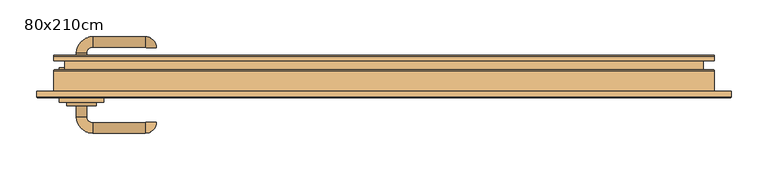
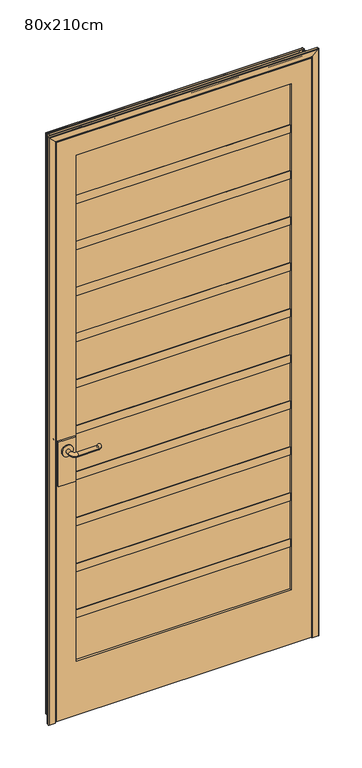
"""IFC4 building model written with IfcOpenShell, lengths in millimetres: door geometry, Porta de Abrir Metálica Quadriculada : 80x210cm."""

from ifc_helpers import new_model, si_unit, point, frame, frame_2d, origin, place, context, project, spatial, polyline, circle_curve, ellipse_curve, trimmed, segment, composite_curve, outline, extrude, source, transform, mapped, element, save
from ifc_brep_helpers import plane_surface, cylinder_surface, revolved_surface, advanced_brep


def door_80x210cm_43d22828(model_context):
    return source(origin(), model_context, "Body", "SolidModel", [
        extrude(outline(composite_curve([segment(trimmed(circle_curve(frame_2d((1050.0, -412.0)), 20.0), [point((1050.0, -432.0))], [point((1050.0, -392.0))], False, "CARTESIAN"), True, "CONTINUOUS"), segment(trimmed(circle_curve(frame_2d((1050.0, -412.0)), 20.0), [point((1050.0, -392.0))], [point((1050.0, -432.0))], False, "CARTESIAN"), True, "CONTINUOUS")], self_intersect=False)), frame((0.0, -53.6, 0.0), z_axis=(0.0, 1.0, 0.0), x_axis=(0.0, 0.0, 1.0)), (0.0, 0.0, 1.0), 4.5929895),
        advanced_brep(
        [(-405.0, -49.0070105, 1050.0), (-419.0, -49.0070105, 1050.0), (-405.0, -33.6, 1050.0), (-419.0, -33.6, 1050.0), (-397.0, -11.6, 1050.0), (-397.0, -25.6, 1050.0), (-325.0, -25.6, 1050.0), (-325.0, -11.6, 1050.0), (-324.0, -26.6, 1050.0), (-310.0, -26.6, 1050.0)],
        [
            (0, 1, circle_curve(frame((-412.0, -49.0070105, 1050.0), z_axis=(0.0, -1.0, 0.0), x_axis=(-1.0, 0.0, 0.0)), 7.0)),
            (1, 0, circle_curve(frame((-412.0, -49.0070105, 1050.0), z_axis=(0.0, -1.0, 0.0), x_axis=(-1.0, 0.0, 0.0)), 7.0)),
            (0, 2),
            (2, 3, circle_curve(frame((-412.0, -33.6, 1050.0), z_axis=(0.0, -1.0, 0.0), x_axis=(-1.0, 0.0, 0.0)), 7.0)),
            (3, 1),
            (3, 2, circle_curve(frame((-412.0, -33.6, 1050.0), z_axis=(0.0, -1.0, 0.0), x_axis=(-1.0, 0.0, 0.0)), 7.0)),
            (4, 3, circle_curve(frame((-397.0, -33.6, 1050.0), z_axis=(0.0, 0.0, 1.0), x_axis=(-1.0, 0.0, 0.0)), 22.0)),
            (2, 5, circle_curve(frame((-397.0, -33.6, 1050.0), z_axis=(0.0, 0.0, -1.0), x_axis=(-1.0, 0.0, 0.0)), 8.0)),
            (5, 4, circle_curve(frame((-397.0, -18.6, 1050.0), z_axis=(-1.0, 0.0, 0.0), x_axis=(0.0, 1.0, 0.0)), 7.0)),
            (4, 5, circle_curve(frame((-397.0, -18.6, 1050.0), z_axis=(-1.0, 0.0, 0.0), x_axis=(0.0, 1.0, 0.0)), 7.0)),
            (5, 6),
            (6, 7, circle_curve(frame((-325.0, -18.6, 1050.0), z_axis=(-1.0, 0.0, 0.0), x_axis=(0.0, 1.0, 0.0)), 7.0)),
            (7, 4),
            (7, 6, circle_curve(frame((-325.0, -18.6, 1050.0), z_axis=(-1.0, 0.0, 0.0), x_axis=(0.0, 1.0, 0.0)), 7.0)),
            (8, 9, circle_curve(frame((-317.0, -26.6, 1050.0), z_axis=(0.0, -1.0, 0.0), x_axis=(1.0, 0.0, 0.0)), 7.0)),
            (9, 8, circle_curve(frame((-317.0, -26.6, 1050.0), z_axis=(0.0, -1.0, 0.0), x_axis=(1.0, 0.0, 0.0)), 7.0)),
            (9, 7, circle_curve(frame((-325.0, -26.6, 1050.0), z_axis=(0.0, 0.0, 1.0), x_axis=(0.0, 1.0, 0.0)), 15.0)),
            (6, 8, circle_curve(frame((-325.0, -26.6, 1050.0), z_axis=(0.0, 0.0, -1.0), x_axis=(0.0, 1.0, 0.0)), 1.0)),
        ],
        [
            plane_surface(frame((-412.0, -49.0070105, 1050.0), z_axis=(0.0, -1.0, 0.0), x_axis=(0.0, 0.0, 1.0))),
            cylinder_surface(frame((-412.0, -49.0070105, 1050.0), z_axis=(0.0, -1.0, 0.0), x_axis=(-1.0, 0.0, 0.0)), 7.0),
            revolved_surface(trimmed(ellipse_curve(frame((-412.0, -33.6, 1050.0), z_axis=(0.0, -1.0, 0.0), x_axis=(-1.0, 0.0, 0.0)), 7.0, 7.0), [point((-405.0, -33.6, 1050.0))], [point((-419.0, -33.6, 1050.0))], True, "CARTESIAN"), (-397.0, -33.6, 1050.0), (0.0, 0.0, -1.0)),
            revolved_surface(trimmed(ellipse_curve(frame((-412.0, -33.6, 1050.0), z_axis=(0.0, -1.0, 0.0), x_axis=(-1.0, 0.0, 0.0)), 7.0, 7.0), [point((-419.0, -33.6, 1050.0))], [point((-405.0, -33.6, 1050.0))], True, "CARTESIAN"), (-397.0, -33.6, 1050.0), (0.0, 0.0, -1.0)),
            cylinder_surface(frame((-397.0, -18.6, 1050.0), z_axis=(-1.0, 0.0, 0.0), x_axis=(0.0, 1.0, 0.0)), 7.0),
            plane_surface(frame((-317.0, -26.6, 1050.0), z_axis=(0.0, -1.0, 0.0), x_axis=(0.0, 0.0, 1.0))),
            revolved_surface(trimmed(ellipse_curve(frame((-325.0, -18.6, 1050.0), z_axis=(-1.0, 0.0, 0.0), x_axis=(0.0, 1.0, 0.0)), 7.0, 7.0), [point((-325.0, -25.6, 1050.0))], [point((-325.0, -11.6, 1050.0))], True, "CARTESIAN"), (-325.0, -26.6, 1050.0), (0.0, 0.0, -1.0)),
            revolved_surface(trimmed(ellipse_curve(frame((-325.0, -18.6, 1050.0), z_axis=(-1.0, 0.0, 0.0), x_axis=(0.0, 1.0, 0.0)), 7.0, 7.0), [point((-325.0, -11.6, 1050.0))], [point((-325.0, -25.6, 1050.0))], True, "CARTESIAN"), (-325.0, -26.6, 1050.0), (0.0, 0.0, -1.0)),
        ],
        [
            (0, [[1, 2]]),
            (1, [[-1, 3, 4, 5]]),
            (1, [[-2, -5, 6, -3]]),
            (2, [[7, -4, 8, 9]]),
            (3, [[-8, -6, -7, 10]]),
            (4, [[-9, 11, 12, 13]]),
            (4, [[-10, -13, 14, -11]]),
            (5, [[15, 16]]),
            (6, [[17, -12, 18, -16]]),
            (7, [[-18, -14, -17, -15]]),
        ],
    ),
        extrude(outline(polyline([(-382.0, -59.6), (-442.0, -59.6), (-442.0, -53.6), (-382.0, -53.6), (-382.0, -59.6)])), frame((0.0, 0.0, 925.0), z_axis=(0.0, 0.0, 1.0), x_axis=(1.0, 0.0, 0.0)), (0.0, 0.0, 1.0), 165.0),
        extrude(outline(composite_curve([segment(trimmed(circle_curve(frame_2d((1050.0, -412.0)), 20.0), [point((1050.0, -432.0))], [point((1050.0, -392.0))], False, "CARTESIAN"), True, "CONTINUOUS"), segment(trimmed(circle_curve(frame_2d((1050.0, -412.0)), 20.0), [point((1050.0, -392.0))], [point((1050.0, -432.0))], False, "CARTESIAN"), True, "CONTINUOUS")], self_intersect=False)), frame((0.0, -105.1929895, 0.0), z_axis=(0.0, 1.0, 0.0), x_axis=(0.0, 0.0, 1.0)), (0.0, 0.0, 1.0), 4.5929895),
        advanced_brep(
        [(-405.0, -105.1929895, 1050.0), (-419.0, -105.1929895, 1050.0), (-419.0, -120.6, 1050.0), (-405.0, -120.6, 1050.0), (-397.0, -142.6, 1050.0), (-397.0, -128.6, 1050.0), (-325.0, -142.6, 1050.0), (-325.0, -128.6, 1050.0), (-324.0, -127.6, 1050.0), (-310.0, -127.6, 1050.0)],
        [
            (0, 1, circle_curve(frame((-412.0, -105.1929895, 1050.0), z_axis=(0.0, 1.0, 0.0), x_axis=(-1.0, 0.0, 0.0)), 7.0)),
            (1, 0, circle_curve(frame((-412.0, -105.1929895, 1050.0), z_axis=(0.0, 1.0, 0.0), x_axis=(-1.0, 0.0, 0.0)), 7.0)),
            (1, 2),
            (2, 3, circle_curve(frame((-412.0, -120.6, 1050.0), z_axis=(0.0, 1.0, 0.0), x_axis=(-1.0, 0.0, 0.0)), 7.0)),
            (3, 0),
            (3, 2, circle_curve(frame((-412.0, -120.6, 1050.0), z_axis=(0.0, 1.0, 0.0), x_axis=(-1.0, 0.0, 0.0)), 7.0)),
            (4, 5, circle_curve(frame((-397.0, -135.6, 1050.0), z_axis=(-1.0, 0.0, 0.0), x_axis=(0.0, -1.0, 0.0)), 7.0)),
            (5, 3, circle_curve(frame((-397.0, -120.6, 1050.0), z_axis=(0.0, 0.0, -1.0), x_axis=(-1.0, 0.0, 0.0)), 8.0)),
            (2, 4, circle_curve(frame((-397.0, -120.6, 1050.0), z_axis=(0.0, 0.0, 1.0), x_axis=(-1.0, 0.0, 0.0)), 22.0)),
            (5, 4, circle_curve(frame((-397.0, -135.6, 1050.0), z_axis=(-1.0, 0.0, 0.0), x_axis=(0.0, -1.0, 0.0)), 7.0)),
            (4, 6),
            (6, 7, circle_curve(frame((-325.0, -135.6, 1050.0), z_axis=(-1.0, 0.0, 0.0), x_axis=(0.0, -1.0, 0.0)), 7.0)),
            (7, 5),
            (7, 6, circle_curve(frame((-325.0, -135.6, 1050.0), z_axis=(-1.0, 0.0, 0.0), x_axis=(0.0, -1.0, 0.0)), 7.0)),
            (8, 9, circle_curve(frame((-317.0, -127.6, 1050.0), z_axis=(0.0, 1.0, 0.0), x_axis=(1.0, 0.0, 0.0)), 7.0)),
            (9, 8, circle_curve(frame((-317.0, -127.6, 1050.0), z_axis=(0.0, 1.0, 0.0), x_axis=(1.0, 0.0, 0.0)), 7.0)),
            (8, 7, circle_curve(frame((-325.0, -127.6, 1050.0), z_axis=(0.0, 0.0, -1.0), x_axis=(0.0, -1.0, 0.0)), 1.0)),
            (6, 9, circle_curve(frame((-325.0, -127.6, 1050.0), z_axis=(0.0, 0.0, 1.0), x_axis=(0.0, -1.0, 0.0)), 15.0)),
        ],
        [
            plane_surface(frame((-412.0, -105.1929895, 1050.0), z_axis=(0.0, 1.0, 0.0), x_axis=(0.0, 0.0, 1.0))),
            cylinder_surface(frame((-412.0, -105.1929895, 1050.0), z_axis=(0.0, 1.0, 0.0), x_axis=(-1.0, 0.0, 0.0)), 7.0),
            revolved_surface(trimmed(ellipse_curve(frame((-412.0, -120.6, 1050.0), z_axis=(0.0, -1.0, 0.0), x_axis=(-1.0, 0.0, 0.0)), 7.0, 7.0), [point((-405.0, -120.6, 1050.0))], [point((-419.0, -120.6, 1050.0))], True, "CARTESIAN"), (-397.0, -120.6, 1050.0), (0.0, 0.0, -1.0)),
            revolved_surface(trimmed(ellipse_curve(frame((-412.0, -120.6, 1050.0), z_axis=(0.0, -1.0, 0.0), x_axis=(-1.0, 0.0, 0.0)), 7.0, 7.0), [point((-419.0, -120.6, 1050.0))], [point((-405.0, -120.6, 1050.0))], True, "CARTESIAN"), (-397.0, -120.6, 1050.0), (0.0, 0.0, -1.0)),
            cylinder_surface(frame((-397.0, -135.6, 1050.0), z_axis=(-1.0, 0.0, 0.0), x_axis=(0.0, -1.0, 0.0)), 7.0),
            plane_surface(frame((-317.0, -127.6, 1050.0), z_axis=(0.0, 1.0, 0.0), x_axis=(0.0, 0.0, 1.0))),
            revolved_surface(trimmed(ellipse_curve(frame((-325.0, -135.6, 1050.0), z_axis=(1.0, 0.0, 0.0), x_axis=(0.0, -1.0, 0.0)), 7.0, 7.0), [point((-325.0, -128.6, 1050.0))], [point((-325.0, -142.6, 1050.0))], True, "CARTESIAN"), (-325.0, -127.6, 1050.0), (0.0, 0.0, -1.0)),
            revolved_surface(trimmed(ellipse_curve(frame((-325.0, -135.6, 1050.0), z_axis=(1.0, 0.0, 0.0), x_axis=(0.0, -1.0, 0.0)), 7.0, 7.0), [point((-325.0, -142.6, 1050.0))], [point((-325.0, -128.6, 1050.0))], True, "CARTESIAN"), (-325.0, -127.6, 1050.0), (0.0, 0.0, -1.0)),
        ],
        [
            (0, [[1, 2]]),
            (1, [[3, 4, 5, -2]]),
            (1, [[-5, 6, -3, -1]]),
            (2, [[7, 8, -4, 9]]),
            (3, [[10, -9, -6, -8]]),
            (4, [[11, 12, 13, -7]]),
            (4, [[-13, 14, -11, -10]]),
            (5, [[15, 16]]),
            (6, [[-15, 17, -12, 18]]),
            (7, [[-16, -18, -14, -17]]),
        ],
    ),
        extrude(outline(polyline([(-382.0, -94.6), (-382.0, -100.6), (-442.0, -100.6), (-442.0, -94.6), (-382.0, -94.6)])), frame((0.0, 0.0, 925.0), z_axis=(0.0, 0.0, 1.0), x_axis=(1.0, 0.0, 0.0)), (0.0, 0.0, 1.0), 165.0),
        extrude(outline(polyline([(377.0, -77.6), (377.0, -86.0), (-377.0, -86.0), (-377.0, -77.6), (377.0, -77.6)])), frame((0.0, 0.0, 253.0), z_axis=(0.0, 0.0, 1.0), x_axis=(1.0, 0.0, 0.0)), (0.0, 0.0, 1.0), 1873.0),
        extrude(outline(polyline([(203.5, -69.6), (203.5, -84.6), (173.5, -84.6), (173.5, -69.6), (203.5, -69.6)])), frame((0.0, 0.0, 253.0), z_axis=(0.0, 0.0, 1.0), x_axis=(1.0, 0.0, 0.0)), (0.0, 0.0, 1.0), 1873.0),
        extrude(outline(polyline([(15.0, -69.6), (15.0, -84.6), (-15.0, -84.6), (-15.0, -69.6), (15.0, -69.6)])), frame((0.0, 0.0, 253.0), z_axis=(0.0, 0.0, 1.0), x_axis=(1.0, 0.0, 0.0)), (0.0, 0.0, 1.0), 1873.0),
        extrude(outline(polyline([(-173.5, -69.6), (-173.5, -84.6), (-203.5, -84.6), (-203.5, -69.6), (-173.5, -69.6)])), frame((0.0, 0.0, 253.0), z_axis=(0.0, 0.0, 1.0), x_axis=(1.0, 0.0, 0.0)), (0.0, 0.0, 1.0), 1873.0),
        extrude(outline(polyline([(377.0, -66.6), (377.0, -87.6), (-377.0, -87.6), (-377.0, -66.6), (377.0, -66.6)])), frame((0.0, 0.0, 1429.9090909), z_axis=(0.0, 0.0, 1.0), x_axis=(1.0, 0.0, 0.0)), (0.0, 0.0, 1.0), 30.0),
        extrude(outline(polyline([(377.0, -66.6), (377.0, -87.6), (-377.0, -87.6), (-377.0, -66.6), (377.0, -66.6)])), frame((0.0, 0.0, 1259.6363636), z_axis=(0.0, 0.0, 1.0), x_axis=(1.0, 0.0, 0.0)), (0.0, 0.0, 1.0), 30.0),
        extrude(outline(polyline([(377.0, -66.6), (377.0, -87.6), (-377.0, -87.6), (-377.0, -66.6), (377.0, -66.6)])), frame((0.0, 0.0, 1089.3636364), z_axis=(0.0, 0.0, 1.0), x_axis=(1.0, 0.0, 0.0)), (0.0, 0.0, 1.0), 30.0),
        extrude(outline(polyline([(377.0, -66.6), (377.0, -87.6), (-377.0, -87.6), (-377.0, -66.6), (377.0, -66.6)])), frame((0.0, 0.0, 919.0909091), z_axis=(0.0, 0.0, 1.0), x_axis=(1.0, 0.0, 0.0)), (0.0, 0.0, 1.0), 30.0),
        extrude(outline(polyline([(377.0, -66.6), (377.0, -87.6), (-377.0, -87.6), (-377.0, -66.6), (377.0, -66.6)])), frame((0.0, 0.0, 748.8181818), z_axis=(0.0, 0.0, 1.0), x_axis=(1.0, 0.0, 0.0)), (0.0, 0.0, 1.0), 30.0),
        extrude(outline(polyline([(377.0, -66.6), (377.0, -87.6), (-377.0, -87.6), (-377.0, -66.6), (377.0, -66.6)])), frame((0.0, 0.0, 578.5454545), z_axis=(0.0, 0.0, 1.0), x_axis=(1.0, 0.0, 0.0)), (0.0, 0.0, 1.0), 30.0),
        extrude(outline(polyline([(377.0, -66.6), (377.0, -87.6), (-377.0, -87.6), (-377.0, -66.6), (377.0, -66.6)])), frame((0.0, 0.0, 408.2727273), z_axis=(0.0, 0.0, 1.0), x_axis=(1.0, 0.0, 0.0)), (0.0, 0.0, 1.0), 30.0),
        extrude(outline(polyline([(377.0, -66.6), (377.0, -87.6), (-377.0, -87.6), (-377.0, -66.6), (377.0, -66.6)])), frame((0.0, 0.0, 1940.7272727), z_axis=(0.0, 0.0, 1.0), x_axis=(1.0, 0.0, 0.0)), (0.0, 0.0, 1.0), 30.0),
        extrude(outline(polyline([(377.0, -66.6), (377.0, -87.6), (-377.0, -87.6), (-377.0, -66.6), (377.0, -66.6)])), frame((0.0, 0.0, 1770.4545455), z_axis=(0.0, 0.0, 1.0), x_axis=(1.0, 0.0, 0.0)), (0.0, 0.0, 1.0), 30.0),
        extrude(outline(polyline([(377.0, -66.6), (377.0, -87.6), (-377.0, -87.6), (-377.0, -66.6), (377.0, -66.6)])), frame((0.0, 0.0, 1600.1818182), z_axis=(0.0, 0.0, 1.0), x_axis=(1.0, 0.0, 0.0)), (0.0, 0.0, 1.0), 30.0),
        extrude(outline(polyline([(2196.0, -447.0), (53.0, -447.0), (53.0, 447.0), (2196.0, 447.0), (2196.0, -447.0)]), holes=[polyline([(2126.0, -377.0), (2126.0, 377.0), (253.0, 377.0), (253.0, -377.0), (2126.0, -377.0)])]), frame((0.0, -94.6, 0.0), z_axis=(0.0, 1.0, 0.0), x_axis=(0.0, 0.0, 1.0)), (0.0, 0.0, 1.0), 35.0),
        advanced_brep(
        [(-435.45, -36.6755478, 50.0), (-433.95, -38.1755478, 50.0), (-433.95, -56.1755478, 50.0), (-435.45, -57.6755478, 50.0), (-448.5, -57.6755478, 50.0), (-449.0, -58.1755478, 50.0), (-449.0, -93.1755478, 50.0), (-450.5, -94.6755478, 50.0), (-471.5, -94.6755478, 50.0), (-473.0, -93.1755478, 50.0), (-473.0, -85.6755478, 50.0), (-472.0, -85.6755478, 50.0), (-472.0, -93.1755478, 50.0), (-471.5, -93.6755478, 50.0), (-450.5, -93.6755478, 50.0), (-450.0, -93.1755478, 50.0), (-450.0, -58.1755478, 50.0), (-448.5, -56.6755478, 50.0), (-435.45, -56.6755478, 50.0), (-434.95, -56.1755478, 50.0), (-434.95, -38.1755478, 50.0), (-435.45, -37.6755478, 50.0), (-448.45, -37.6755478, 50.0), (-448.95, -38.1755478, 50.0), (-448.95, -44.6755478, 50.0), (-449.95, -44.6755478, 50.0), (-449.95, -38.1755478, 50.0), (-448.45, -36.6755478, 50.0), (-448.45, -36.6755478, 2198.45), (-435.45, -36.6755478, 2185.45), (-449.95, -38.1755478, 2199.95), (-449.95, -44.6755478, 2199.95), (-448.95, -44.6755478, 2198.95), (-448.95, -38.1755478, 2198.95), (-448.45, -37.6755478, 2198.45), (-435.45, -37.6755478, 2185.45), (-434.95, -38.1755478, 2184.95), (-434.95, -56.1755478, 2184.95), (-435.45, -56.6755478, 2185.45), (-448.5, -56.6755478, 2198.5), (-450.0, -58.1755478, 2200.0), (-450.0, -93.1755478, 2200.0), (-450.5, -93.6755478, 2200.5), (-471.5, -93.6755478, 2221.5), (-472.0, -93.1755478, 2222.0), (-472.0, -85.6755478, 2222.0), (-473.0, -85.6755478, 2223.0), (-473.0, -93.1755478, 2223.0), (-471.5, -94.6755478, 2221.5), (-450.5, -94.6755478, 2200.5), (-449.0, -93.1755478, 2199.0), (-449.0, -58.1755478, 2199.0), (-448.5, -57.6755478, 2198.5), (-435.45, -57.6755478, 2185.45), (-433.95, -56.1755478, 2183.95), (-433.95, -38.1755478, 2183.95), (435.45, -36.6755478, 50.0), (448.45, -36.6755478, 50.0), (449.95, -38.1755478, 50.0), (449.95, -44.6755478, 50.0), (448.95, -44.6755478, 50.0), (448.95, -38.1755478, 50.0), (448.45, -37.6755478, 50.0), (435.45, -37.6755478, 50.0), (434.95, -38.1755478, 50.0), (434.95, -56.1755478, 50.0), (435.45, -56.6755478, 50.0), (448.5, -56.6755478, 50.0), (450.0, -58.1755478, 50.0), (450.0, -93.1755478, 50.0), (450.5, -93.6755478, 50.0), (471.5, -93.6755478, 50.0), (472.0, -93.1755478, 50.0), (472.0, -85.6755478, 50.0), (473.0, -85.6755478, 50.0), (473.0, -93.1755478, 50.0), (471.5, -94.6755478, 50.0), (450.5, -94.6755478, 50.0), (449.0, -93.1755478, 50.0), (449.0, -58.1755478, 50.0), (448.5, -57.6755478, 50.0), (435.45, -57.6755478, 50.0), (433.95, -56.1755478, 50.0), (433.95, -38.1755478, 50.0), (435.45, -36.6755478, 2185.45), (433.95, -38.1755478, 2183.95), (433.95, -56.1755478, 2183.95), (435.45, -57.6755478, 2185.45), (448.5, -57.6755478, 2198.5), (449.0, -58.1755478, 2199.0), (449.0, -93.1755478, 2199.0), (450.5, -94.6755478, 2200.5), (471.5, -94.6755478, 2221.5), (473.0, -93.1755478, 2223.0), (473.0, -85.6755478, 2223.0), (472.0, -85.6755478, 2222.0), (472.0, -93.1755478, 2222.0), (471.5, -93.6755478, 2221.5), (450.5, -93.6755478, 2200.5), (450.0, -93.1755478, 2200.0), (450.0, -58.1755478, 2200.0), (448.5, -56.6755478, 2198.5), (435.45, -56.6755478, 2185.45), (434.95, -56.1755478, 2184.95), (434.95, -38.1755478, 2184.95), (435.45, -37.6755478, 2185.45), (448.45, -37.6755478, 2198.45), (448.95, -38.1755478, 2198.95), (448.95, -44.6755478, 2198.95), (449.95, -44.6755478, 2199.95), (449.95, -38.1755478, 2199.95), (448.45, -36.6755478, 2198.45)],
        [
            (0, 1, circle_curve(frame((-435.45, -38.1755478, 50.0), z_axis=(0.0, 0.0, -1.0), x_axis=(1.0, 0.0, 0.0)), 1.5)),
            (1, 2),
            (2, 3, circle_curve(frame((-435.45, -56.1755478, 50.0), z_axis=(0.0, 0.0, -1.0), x_axis=(1.0, 0.0, 0.0)), 1.5)),
            (3, 4),
            (4, 5, circle_curve(frame((-448.5, -58.1755478, 50.0), z_axis=(0.0, 0.0, 1.0), x_axis=(1.0, 0.0, 0.0)), 0.5)),
            (5, 6),
            (6, 7, circle_curve(frame((-450.5, -93.1755478, 50.0), z_axis=(0.0, 0.0, -1.0), x_axis=(1.0, 0.0, 0.0)), 1.5)),
            (7, 8),
            (8, 9, circle_curve(frame((-471.5, -93.1755478, 50.0), z_axis=(0.0, 0.0, -1.0), x_axis=(1.0, 0.0, 0.0)), 1.5)),
            (9, 10),
            (10, 11),
            (11, 12),
            (12, 13, circle_curve(frame((-471.5, -93.1755478, 50.0), z_axis=(0.0, 0.0, 1.0), x_axis=(1.0, 0.0, 0.0)), 0.5)),
            (13, 14),
            (14, 15, circle_curve(frame((-450.5, -93.1755478, 50.0), z_axis=(0.0, 0.0, 1.0), x_axis=(1.0, 0.0, 0.0)), 0.5)),
            (15, 16),
            (16, 17, circle_curve(frame((-448.5, -58.1755478, 50.0), z_axis=(0.0, 0.0, -1.0), x_axis=(1.0, 0.0, 0.0)), 1.5)),
            (17, 18),
            (18, 19, circle_curve(frame((-435.45, -56.1755478, 50.0), z_axis=(0.0, 0.0, 1.0), x_axis=(1.0, 0.0, 0.0)), 0.5)),
            (19, 20),
            (20, 21, circle_curve(frame((-435.45, -38.1755478, 50.0), z_axis=(0.0, 0.0, 1.0), x_axis=(1.0, 0.0, 0.0)), 0.5)),
            (21, 22),
            (22, 23, circle_curve(frame((-448.45, -38.1755478, 50.0), z_axis=(0.0, 0.0, 1.0), x_axis=(1.0, 0.0, 0.0)), 0.5)),
            (23, 24),
            (24, 25),
            (25, 26),
            (26, 27, circle_curve(frame((-448.45, -38.1755478, 50.0), z_axis=(0.0, 0.0, -1.0), x_axis=(1.0, 0.0, 0.0)), 1.5)),
            (27, 0),
            (27, 28),
            (28, 29),
            (29, 0),
            (26, 30),
            (30, 28, ellipse_curve(frame((-448.45, -38.1755478, 2198.45), z_axis=(-0.7071067811865475, 0.0, -0.7071067811865475), x_axis=(0.7071067811865474, 0.0, -0.7071067811865476)), 2.1213203, 1.5)),
            (25, 31),
            (31, 30),
            (24, 32),
            (32, 31),
            (23, 33),
            (33, 32),
            (22, 34),
            (34, 33, ellipse_curve(frame((-448.45, -38.1755478, 2198.45), z_axis=(0.7071067811865475, 0.0, 0.7071067811865475), x_axis=(-0.7071067811865474, 0.0, 0.7071067811865476)), 0.7071068, 0.5)),
            (21, 35),
            (35, 34),
            (20, 36),
            (36, 35, ellipse_curve(frame((-435.45, -38.1755478, 2185.45), z_axis=(0.7071067811865475, 0.0, 0.7071067811865475), x_axis=(-0.7071067811865474, 0.0, 0.7071067811865476)), 0.7071068, 0.5)),
            (19, 37),
            (37, 36),
            (18, 38),
            (38, 37, ellipse_curve(frame((-435.45, -56.1755478, 2185.45), z_axis=(0.7071067811865475, 0.0, 0.7071067811865475), x_axis=(-0.7071067811865474, 0.0, 0.7071067811865476)), 0.7071068, 0.5)),
            (17, 39),
            (39, 38),
            (16, 40),
            (40, 39, ellipse_curve(frame((-448.5, -58.1755478, 2198.5), z_axis=(-0.7071067811865475, 0.0, -0.7071067811865475), x_axis=(0.7071067811865474, 0.0, -0.7071067811865476)), 2.1213203, 1.5)),
            (15, 41),
            (41, 40),
            (14, 42),
            (42, 41, ellipse_curve(frame((-450.5, -93.1755478, 2200.5), z_axis=(0.7071067811865475, 0.0, 0.7071067811865475), x_axis=(-0.7071067811865474, 0.0, 0.7071067811865476)), 0.7071068, 0.5)),
            (13, 43),
            (43, 42),
            (12, 44),
            (44, 43, ellipse_curve(frame((-471.5, -93.1755478, 2221.5), z_axis=(0.7071067811865475, 0.0, 0.7071067811865475), x_axis=(-0.7071067811865474, 0.0, 0.7071067811865476)), 0.7071068, 0.5)),
            (11, 45),
            (45, 44),
            (10, 46),
            (46, 45),
            (9, 47),
            (47, 46),
            (8, 48),
            (48, 47, ellipse_curve(frame((-471.5, -93.1755478, 2221.5), z_axis=(-0.7071067811865475, 0.0, -0.7071067811865475), x_axis=(0.7071067811865474, 0.0, -0.7071067811865476)), 2.1213203, 1.5)),
            (7, 49),
            (49, 48),
            (6, 50),
            (50, 49, ellipse_curve(frame((-450.5, -93.1755478, 2200.5), z_axis=(-0.7071067811865475, 0.0, -0.7071067811865475), x_axis=(0.7071067811865474, 0.0, -0.7071067811865476)), 2.1213203, 1.5)),
            (5, 51),
            (51, 50),
            (4, 52),
            (52, 51, ellipse_curve(frame((-448.5, -58.1755478, 2198.5), z_axis=(0.7071067811865475, 0.0, 0.7071067811865475), x_axis=(-0.7071067811865474, 0.0, 0.7071067811865476)), 0.7071068, 0.5)),
            (3, 53),
            (53, 52),
            (2, 54),
            (54, 53, ellipse_curve(frame((-435.45, -56.1755478, 2185.45), z_axis=(-0.7071067811865475, 0.0, -0.7071067811865475), x_axis=(0.7071067811865474, 0.0, -0.7071067811865476)), 2.1213203, 1.5)),
            (1, 55),
            (55, 54),
            (29, 55, ellipse_curve(frame((-435.45, -38.1755478, 2185.45), z_axis=(-0.7071067811865475, 0.0, -0.7071067811865475), x_axis=(0.7071067811865474, 0.0, -0.7071067811865476)), 2.1213203, 1.5)),
            (56, 57),
            (57, 58, circle_curve(frame((448.45, -38.1755478, 50.0), z_axis=(0.0, 0.0, -1.0), x_axis=(-1.0, 0.0, 0.0)), 1.5)),
            (58, 59),
            (59, 60),
            (60, 61),
            (61, 62, circle_curve(frame((448.45, -38.1755478, 50.0), z_axis=(0.0, 0.0, 1.0), x_axis=(-1.0, 0.0, 0.0)), 0.5)),
            (62, 63),
            (63, 64, circle_curve(frame((435.45, -38.1755478, 50.0), z_axis=(0.0, 0.0, 1.0), x_axis=(-1.0, 0.0, 0.0)), 0.5)),
            (64, 65),
            (65, 66, circle_curve(frame((435.45, -56.1755478, 50.0), z_axis=(0.0, 0.0, 1.0), x_axis=(-1.0, 0.0, 0.0)), 0.5)),
            (66, 67),
            (67, 68, circle_curve(frame((448.5, -58.1755478, 50.0), z_axis=(0.0, 0.0, -1.0), x_axis=(-1.0, 0.0, 0.0)), 1.5)),
            (68, 69),
            (69, 70, circle_curve(frame((450.5, -93.1755478, 50.0), z_axis=(0.0, 0.0, 1.0), x_axis=(-1.0, 0.0, 0.0)), 0.5)),
            (70, 71),
            (71, 72, circle_curve(frame((471.5, -93.1755478, 50.0), z_axis=(0.0, 0.0, 1.0), x_axis=(-1.0, 0.0, 0.0)), 0.5)),
            (72, 73),
            (73, 74),
            (74, 75),
            (75, 76, circle_curve(frame((471.5, -93.1755478, 50.0), z_axis=(0.0, 0.0, -1.0), x_axis=(-1.0, 0.0, 0.0)), 1.5)),
            (76, 77),
            (77, 78, circle_curve(frame((450.5, -93.1755478, 50.0), z_axis=(0.0, 0.0, -1.0), x_axis=(-1.0, 0.0, 0.0)), 1.5)),
            (78, 79),
            (79, 80, circle_curve(frame((448.5, -58.1755478, 50.0), z_axis=(0.0, 0.0, 1.0), x_axis=(-1.0, 0.0, 0.0)), 0.5)),
            (80, 81),
            (81, 82, circle_curve(frame((435.45, -56.1755478, 50.0), z_axis=(0.0, 0.0, -1.0), x_axis=(-1.0, 0.0, 0.0)), 1.5)),
            (82, 83),
            (83, 56, circle_curve(frame((435.45, -38.1755478, 50.0), z_axis=(0.0, 0.0, -1.0), x_axis=(-1.0, 0.0, 0.0)), 1.5)),
            (84, 56),
            (83, 85),
            (85, 84, ellipse_curve(frame((435.45, -38.1755478, 2185.45), z_axis=(0.7071067811865475, 0.0, -0.7071067811865475), x_axis=(0.7071067811865474, 0.0, 0.7071067811865476)), 2.1213203, 1.5)),
            (82, 86),
            (86, 85),
            (81, 87),
            (87, 86, ellipse_curve(frame((435.45, -56.1755478, 2185.45), z_axis=(0.7071067811865475, 0.0, -0.7071067811865475), x_axis=(0.7071067811865474, 0.0, 0.7071067811865476)), 2.1213203, 1.5)),
            (80, 88),
            (88, 87),
            (79, 89),
            (89, 88, ellipse_curve(frame((448.5, -58.1755478, 2198.5), z_axis=(-0.7071067811865475, 0.0, 0.7071067811865475), x_axis=(-0.7071067811865474, 0.0, -0.7071067811865476)), 0.7071068, 0.5)),
            (78, 90),
            (90, 89),
            (77, 91),
            (91, 90, ellipse_curve(frame((450.5, -93.1755478, 2200.5), z_axis=(0.7071067811865475, 0.0, -0.7071067811865475), x_axis=(0.7071067811865474, 0.0, 0.7071067811865476)), 2.1213203, 1.5)),
            (76, 92),
            (92, 91),
            (75, 93),
            (93, 92, ellipse_curve(frame((471.5, -93.1755478, 2221.5), z_axis=(0.7071067811865475, 0.0, -0.7071067811865475), x_axis=(0.7071067811865474, 0.0, 0.7071067811865476)), 2.1213203, 1.5)),
            (74, 94),
            (94, 93),
            (73, 95),
            (95, 94),
            (72, 96),
            (96, 95),
            (71, 97),
            (97, 96, ellipse_curve(frame((471.5, -93.1755478, 2221.5), z_axis=(-0.7071067811865475, 0.0, 0.7071067811865475), x_axis=(-0.7071067811865474, 0.0, -0.7071067811865476)), 0.7071068, 0.5)),
            (70, 98),
            (98, 97),
            (69, 99),
            (99, 98, ellipse_curve(frame((450.5, -93.1755478, 2200.5), z_axis=(-0.7071067811865475, 0.0, 0.7071067811865475), x_axis=(-0.7071067811865474, 0.0, -0.7071067811865476)), 0.7071068, 0.5)),
            (68, 100),
            (100, 99),
            (67, 101),
            (101, 100, ellipse_curve(frame((448.5, -58.1755478, 2198.5), z_axis=(0.7071067811865475, 0.0, -0.7071067811865475), x_axis=(0.7071067811865474, 0.0, 0.7071067811865476)), 2.1213203, 1.5)),
            (66, 102),
            (102, 101),
            (65, 103),
            (103, 102, ellipse_curve(frame((435.45, -56.1755478, 2185.45), z_axis=(-0.7071067811865475, 0.0, 0.7071067811865475), x_axis=(-0.7071067811865474, 0.0, -0.7071067811865476)), 0.7071068, 0.5)),
            (64, 104),
            (104, 103),
            (63, 105),
            (105, 104, ellipse_curve(frame((435.45, -38.1755478, 2185.45), z_axis=(-0.7071067811865475, 0.0, 0.7071067811865475), x_axis=(-0.7071067811865474, 0.0, -0.7071067811865476)), 0.7071068, 0.5)),
            (62, 106),
            (106, 105),
            (61, 107),
            (107, 106, ellipse_curve(frame((448.45, -38.1755478, 2198.45), z_axis=(-0.7071067811865475, 0.0, 0.7071067811865475), x_axis=(-0.7071067811865474, 0.0, -0.7071067811865476)), 0.7071068, 0.5)),
            (60, 108),
            (108, 107),
            (59, 109),
            (109, 108),
            (58, 110),
            (110, 109),
            (57, 111),
            (111, 110, ellipse_curve(frame((448.45, -38.1755478, 2198.45), z_axis=(0.7071067811865475, 0.0, -0.7071067811865475), x_axis=(0.7071067811865474, 0.0, 0.7071067811865476)), 2.1213203, 1.5)),
            (84, 111),
            (28, 111),
            (84, 29),
            (30, 110),
            (31, 109),
            (32, 108),
            (33, 107),
            (34, 106),
            (35, 105),
            (36, 104),
            (37, 103),
            (38, 102),
            (39, 101),
            (40, 100),
            (41, 99),
            (42, 98),
            (43, 97),
            (44, 96),
            (45, 95),
            (46, 94),
            (47, 93),
            (48, 92),
            (49, 91),
            (50, 90),
            (51, 89),
            (52, 88),
            (53, 87),
            (54, 86),
            (55, 85),
        ],
        [
            plane_surface(frame((-450.0, -34.5578163, 50.0), z_axis=(0.0, 0.0, -1.0), x_axis=(1.0, 0.0, 0.0))),
            plane_surface(frame((-435.45, -36.6755478, 50.0), z_axis=(0.0, 1.0, 0.0), x_axis=(0.0, 0.0, 1.0))),
            cylinder_surface(frame((-448.45, -38.1755478, 50.0), z_axis=(0.0, 0.0, -1.0), x_axis=(1.0, 0.0, 0.0)), 1.5),
            plane_surface(frame((-449.95, -38.1755478, 50.0), z_axis=(-1.0, 0.0, 0.0), x_axis=(0.0, 0.0, 1.0))),
            plane_surface(frame((-449.95, -44.6755478, 50.0), z_axis=(0.0, -1.0, 0.0), x_axis=(0.0, 0.0, 1.0))),
            plane_surface(frame((-448.95, -44.6755478, 50.0), z_axis=(1.0, 0.0, 0.0), x_axis=(0.0, 0.0, 1.0))),
            revolved_surface(polyline([(-447.95, -38.1755478, 2198.950000013303), (-447.95, -38.1755478, 50.0)]), (-448.45, -38.1755478, 50.0), (0.0, 0.0, 1.0)),
            plane_surface(frame((-448.45, -37.6755478, 50.0), z_axis=(0.0, -1.0, 0.0), x_axis=(0.0, 0.0, 1.0))),
            revolved_surface(polyline([(-434.95, -38.1755478, 2185.950000013303), (-434.95, -38.1755478, 50.0)]), (-435.45, -38.1755478, 50.0), (0.0, 0.0, 1.0)),
            plane_surface(frame((-434.95, -38.1755478, 50.0), z_axis=(-1.0, 0.0, 0.0), x_axis=(0.0, 0.0, 1.0))),
            revolved_surface(polyline([(-434.95, -56.1755478, 2185.950000013303), (-434.95, -56.1755478, 50.0)]), (-435.45, -56.1755478, 50.0), (0.0, 0.0, 1.0)),
            plane_surface(frame((-435.45, -56.6755478, 50.0), z_axis=(0.0, 1.0, 0.0), x_axis=(0.0, 0.0, 1.0))),
            cylinder_surface(frame((-448.5, -58.1755478, 50.0), z_axis=(0.0, 0.0, -1.0), x_axis=(1.0, 0.0, 0.0)), 1.5),
            plane_surface(frame((-450.0, -58.1755478, 50.0), z_axis=(-1.0, 0.0, 0.0), x_axis=(0.0, 0.0, 1.0))),
            revolved_surface(polyline([(-450.0, -93.1755478, 2201.000000013303), (-450.0, -93.1755478, 50.0)]), (-450.5, -93.1755478, 50.0), (0.0, 0.0, 1.0)),
            plane_surface(frame((-450.5, -93.6755478, 50.0), z_axis=(0.0, 1.0, 0.0), x_axis=(0.0, 0.0, 1.0))),
            revolved_surface(polyline([(-471.0, -93.1755478, 2222.000000013303), (-471.0, -93.1755478, 50.0)]), (-471.5, -93.1755478, 50.0), (0.0, 0.0, 1.0)),
            plane_surface(frame((-472.0, -93.1755478, 50.0), z_axis=(1.0, 0.0, 0.0), x_axis=(0.0, 0.0, 1.0))),
            plane_surface(frame((-472.0, -85.6755478, 50.0), z_axis=(0.0, 1.0, 0.0), x_axis=(0.0, 0.0, 1.0))),
            plane_surface(frame((-473.0, -85.6755478, 50.0), z_axis=(-1.0, 0.0, 0.0), x_axis=(0.0, 0.0, 1.0))),
            cylinder_surface(frame((-471.5, -93.1755478, 50.0), z_axis=(0.0, 0.0, -1.0), x_axis=(1.0, 0.0, 0.0)), 1.5),
            plane_surface(frame((-471.5, -94.6755478, 50.0), z_axis=(0.0, -1.0, 0.0), x_axis=(0.0, 0.0, 1.0))),
            cylinder_surface(frame((-450.5, -93.1755478, 50.0), z_axis=(0.0, 0.0, -1.0), x_axis=(1.0, 0.0, 0.0)), 1.5),
            plane_surface(frame((-449.0, -93.1755478, 50.0), z_axis=(1.0, 0.0, 0.0), x_axis=(0.0, 0.0, 1.0))),
            revolved_surface(polyline([(-448.0, -58.1755478, 2199.000000013303), (-448.0, -58.1755478, 50.0)]), (-448.5, -58.1755478, 50.0), (0.0, 0.0, 1.0)),
            plane_surface(frame((-448.5, -57.6755478, 50.0), z_axis=(0.0, -1.0, 0.0), x_axis=(0.0, 0.0, 1.0))),
            cylinder_surface(frame((-435.45, -56.1755478, 50.0), z_axis=(0.0, 0.0, -1.0), x_axis=(1.0, 0.0, 0.0)), 1.5),
            plane_surface(frame((-433.95, -56.1755478, 50.0), z_axis=(1.0, 0.0, 0.0), x_axis=(0.0, 0.0, 1.0))),
            cylinder_surface(frame((-435.45, -38.1755478, 50.0), z_axis=(0.0, 0.0, -1.0), x_axis=(1.0, 0.0, 0.0)), 1.5),
            plane_surface(frame((450.0, -34.5578163, 50.0), z_axis=(0.0, 0.0, -1.0), x_axis=(-1.0, 0.0, 0.0))),
            cylinder_surface(frame((435.45, -38.1755478, 2200.0), z_axis=(0.0, 0.0, 1.0), x_axis=(-1.0, 0.0, 0.0)), 1.5),
            plane_surface(frame((433.95, -56.1755478, 2183.95), z_axis=(-1.0, 0.0, 0.0), x_axis=(0.0, 0.0, -1.0))),
            cylinder_surface(frame((435.45, -56.1755478, 2200.0), z_axis=(0.0, 0.0, 1.0), x_axis=(-1.0, 0.0, 0.0)), 1.5),
            plane_surface(frame((448.5, -57.6755478, 2198.5), z_axis=(0.0, -1.0, 0.0), x_axis=(0.0, 0.0, -1.0))),
            revolved_surface(polyline([(448.0, -58.1755478, 50.0), (448.0, -58.1755478, 2199.000000013303)]), (448.5, -58.1755478, 2200.0), (0.0, 0.0, -1.0)),
            plane_surface(frame((449.0, -93.1755478, 2199.0), z_axis=(-1.0, 0.0, 0.0), x_axis=(0.0, 0.0, -1.0))),
            cylinder_surface(frame((450.5, -93.1755478, 2200.0), z_axis=(0.0, 0.0, 1.0), x_axis=(-1.0, 0.0, 0.0)), 1.5),
            plane_surface(frame((471.5, -94.6755478, 2221.5), z_axis=(0.0, -1.0, 0.0), x_axis=(0.0, 0.0, -1.0))),
            cylinder_surface(frame((471.5, -93.1755478, 2200.0), z_axis=(0.0, 0.0, 1.0), x_axis=(-1.0, 0.0, 0.0)), 1.5),
            plane_surface(frame((473.0, -85.6755478, 2223.0), z_axis=(1.0, 0.0, 0.0), x_axis=(0.0, 0.0, -1.0))),
            plane_surface(frame((472.0, -85.6755478, 2222.0), z_axis=(0.0, 1.0, 0.0), x_axis=(0.0, 0.0, -1.0))),
            plane_surface(frame((472.0, -93.1755478, 2222.0), z_axis=(-1.0, 0.0, 0.0), x_axis=(0.0, 0.0, -1.0))),
            revolved_surface(polyline([(471.0, -93.1755478, 50.0), (471.0, -93.1755478, 2222.000000013303)]), (471.5, -93.1755478, 2200.0), (0.0, 0.0, -1.0)),
            plane_surface(frame((450.5, -93.6755478, 2200.5), z_axis=(0.0, 1.0, 0.0), x_axis=(0.0, 0.0, -1.0))),
            revolved_surface(polyline([(450.0, -93.1755478, 50.0), (450.0, -93.1755478, 2201.000000013303)]), (450.5, -93.1755478, 2200.0), (0.0, 0.0, -1.0)),
            plane_surface(frame((450.0, -58.1755478, 2200.0), z_axis=(1.0, 0.0, 0.0), x_axis=(0.0, 0.0, -1.0))),
            cylinder_surface(frame((448.5, -58.1755478, 2200.0), z_axis=(0.0, 0.0, 1.0), x_axis=(-1.0, 0.0, 0.0)), 1.5),
            plane_surface(frame((435.45, -56.6755478, 2185.45), z_axis=(0.0, 1.0, 0.0), x_axis=(0.0, 0.0, -1.0))),
            revolved_surface(polyline([(434.95, -56.1755478, 50.0), (434.95, -56.1755478, 2185.950000013303)]), (435.45, -56.1755478, 2200.0), (0.0, 0.0, -1.0)),
            plane_surface(frame((434.95, -38.1755478, 2184.95), z_axis=(1.0, 0.0, 0.0), x_axis=(0.0, 0.0, -1.0))),
            revolved_surface(polyline([(434.95, -38.1755478, 50.0), (434.95, -38.1755478, 2185.950000013303)]), (435.45, -38.1755478, 2200.0), (0.0, 0.0, -1.0)),
            plane_surface(frame((448.45, -37.6755478, 2198.45), z_axis=(0.0, -1.0, 0.0), x_axis=(0.0, 0.0, -1.0))),
            revolved_surface(polyline([(447.95, -38.1755478, 50.0), (447.95, -38.1755478, 2198.950000013303)]), (448.45, -38.1755478, 2200.0), (0.0, 0.0, -1.0)),
            plane_surface(frame((448.95, -44.6755478, 2198.95), z_axis=(-1.0, 0.0, 0.0), x_axis=(0.0, 0.0, -1.0))),
            plane_surface(frame((449.95, -44.6755478, 2199.95), z_axis=(0.0, -1.0, 0.0), x_axis=(0.0, 0.0, -1.0))),
            plane_surface(frame((449.95, -38.1755478, 2199.95), z_axis=(1.0, 0.0, 0.0), x_axis=(0.0, 0.0, -1.0))),
            cylinder_surface(frame((448.45, -38.1755478, 2200.0), z_axis=(0.0, 0.0, 1.0), x_axis=(-1.0, 0.0, 0.0)), 1.5),
            plane_surface(frame((435.45, -36.6755478, 2185.45), z_axis=(0.0, 1.0, 0.0), x_axis=(0.0, 0.0, -1.0))),
            plane_surface(frame((-435.45, -36.6755478, 2185.45), z_axis=(0.0, 1.0, 0.0), x_axis=(1.0, 0.0, 0.0))),
            cylinder_surface(frame((-450.0, -38.1755478, 2198.45), z_axis=(-1.0, 0.0, 0.0), x_axis=(0.0, 0.0, -1.0)), 1.5),
            plane_surface(frame((-449.95, -38.1755478, 2199.95), z_axis=(0.0, 0.0, 1.0), x_axis=(1.0, 0.0, 0.0))),
            plane_surface(frame((-449.95, -44.6755478, 2199.95), z_axis=(0.0, -1.0, 0.0), x_axis=(1.0, 0.0, 0.0))),
            plane_surface(frame((-448.95, -44.6755478, 2198.95), z_axis=(0.0, 0.0, -1.0), x_axis=(1.0, 0.0, 0.0))),
            revolved_surface(polyline([(448.9500000133031, -38.1755478, 2197.95), (-448.9500000133031, -38.1755478, 2197.95)]), (-450.0, -38.1755478, 2198.45), (1.0, 0.0, 0.0)),
            plane_surface(frame((-448.45, -37.6755478, 2198.45), z_axis=(0.0, -1.0, 0.0), x_axis=(1.0, 0.0, 0.0))),
            revolved_surface(polyline([(435.9500000133031, -38.1755478, 2184.95), (-435.9500000133031, -38.1755478, 2184.95)]), (-450.0, -38.1755478, 2185.45), (1.0, 0.0, 0.0)),
            plane_surface(frame((-434.95, -38.1755478, 2184.95), z_axis=(0.0, 0.0, 1.0), x_axis=(1.0, 0.0, 0.0))),
            revolved_surface(polyline([(435.9500000133031, -56.1755478, 2184.95), (-435.9500000133031, -56.1755478, 2184.95)]), (-450.0, -56.1755478, 2185.45), (1.0, 0.0, 0.0)),
            plane_surface(frame((-435.45, -56.6755478, 2185.45), z_axis=(0.0, 1.0, 0.0), x_axis=(1.0, 0.0, 0.0))),
            cylinder_surface(frame((-450.0, -58.1755478, 2198.5), z_axis=(-1.0, 0.0, 0.0), x_axis=(0.0, 0.0, -1.0)), 1.5),
            plane_surface(frame((-450.0, -58.1755478, 2200.0), z_axis=(0.0, 0.0, 1.0), x_axis=(1.0, 0.0, 0.0))),
            revolved_surface(polyline([(451.00000001330307, -93.1755478, 2200.0), (-451.0000000133031, -93.1755478, 2200.0)]), (-450.0, -93.1755478, 2200.5), (1.0, 0.0, 0.0)),
            plane_surface(frame((-450.5, -93.6755478, 2200.5), z_axis=(0.0, 1.0, 0.0), x_axis=(1.0, 0.0, 0.0))),
            revolved_surface(polyline([(472.00000001330307, -93.1755478, 2221.0), (-472.0000000133031, -93.1755478, 2221.0)]), (-450.0, -93.1755478, 2221.5), (1.0, 0.0, 0.0)),
            plane_surface(frame((-472.0, -93.1755478, 2222.0), z_axis=(0.0, 0.0, -1.0), x_axis=(1.0, 0.0, 0.0))),
            plane_surface(frame((-472.0, -85.6755478, 2222.0), z_axis=(0.0, 1.0, 0.0), x_axis=(1.0, 0.0, 0.0))),
            plane_surface(frame((-473.0, -85.6755478, 2223.0), z_axis=(0.0, 0.0, 1.0), x_axis=(1.0, 0.0, 0.0))),
            cylinder_surface(frame((-450.0, -93.1755478, 2221.5), z_axis=(-1.0, 0.0, 0.0), x_axis=(0.0, 0.0, -1.0)), 1.5),
            plane_surface(frame((-471.5, -94.6755478, 2221.5), z_axis=(0.0, -1.0, 0.0), x_axis=(1.0, 0.0, 0.0))),
            cylinder_surface(frame((-450.0, -93.1755478, 2200.5), z_axis=(-1.0, 0.0, 0.0), x_axis=(0.0, 0.0, -1.0)), 1.5),
            plane_surface(frame((-449.0, -93.1755478, 2199.0), z_axis=(0.0, 0.0, -1.0), x_axis=(1.0, 0.0, 0.0))),
            revolved_surface(polyline([(449.00000001330307, -58.1755478, 2198.0), (-449.0000000133031, -58.1755478, 2198.0)]), (-450.0, -58.1755478, 2198.5), (1.0, 0.0, 0.0)),
            plane_surface(frame((-448.5, -57.6755478, 2198.5), z_axis=(0.0, -1.0, 0.0), x_axis=(1.0, 0.0, 0.0))),
            cylinder_surface(frame((-450.0, -56.1755478, 2185.45), z_axis=(-1.0, 0.0, 0.0), x_axis=(0.0, 0.0, -1.0)), 1.5),
            plane_surface(frame((-433.95, -56.1755478, 2183.95), z_axis=(0.0, 0.0, -1.0), x_axis=(1.0, 0.0, 0.0))),
            cylinder_surface(frame((-450.0, -38.1755478, 2185.45), z_axis=(-1.0, 0.0, 0.0), x_axis=(0.0, 0.0, -1.0)), 1.5),
        ],
        [
            (0, [[1, 2, 3, 4, 5, 6, 7, 8, 9, 10, 11, 12, 13, 14, 15, 16, 17, 18, 19, 20, 21, 22, 23, 24, 25, 26, 27, 28]]),
            (1, [[29, 30, 31, -28]]),
            (2, [[32, 33, -29, -27]]),
            (3, [[34, 35, -32, -26]]),
            (4, [[36, 37, -34, -25]]),
            (5, [[38, 39, -36, -24]]),
            (6, [[40, 41, -38, -23]]),
            (7, [[42, 43, -40, -22]]),
            (8, [[44, 45, -42, -21]]),
            (9, [[46, 47, -44, -20]]),
            (10, [[48, 49, -46, -19]]),
            (11, [[50, 51, -48, -18]]),
            (12, [[52, 53, -50, -17]]),
            (13, [[54, 55, -52, -16]]),
            (14, [[56, 57, -54, -15]]),
            (15, [[58, 59, -56, -14]]),
            (16, [[60, 61, -58, -13]]),
            (17, [[62, 63, -60, -12]]),
            (18, [[64, 65, -62, -11]]),
            (19, [[66, 67, -64, -10]]),
            (20, [[68, 69, -66, -9]]),
            (21, [[70, 71, -68, -8]]),
            (22, [[72, 73, -70, -7]]),
            (23, [[74, 75, -72, -6]]),
            (24, [[76, 77, -74, -5]]),
            (25, [[78, 79, -76, -4]]),
            (26, [[80, 81, -78, -3]]),
            (27, [[82, 83, -80, -2]]),
            (28, [[-31, 84, -82, -1]]),
            (29, [[85, 86, 87, 88, 89, 90, 91, 92, 93, 94, 95, 96, 97, 98, 99, 100, 101, 102, 103, 104, 105, 106, 107, 108, 109, 110, 111, 112]]),
            (30, [[113, -112, 114, 115]]),
            (31, [[-114, -111, 116, 117]]),
            (32, [[-116, -110, 118, 119]]),
            (33, [[-118, -109, 120, 121]]),
            (34, [[-120, -108, 122, 123]]),
            (35, [[-122, -107, 124, 125]]),
            (36, [[-124, -106, 126, 127]]),
            (37, [[-126, -105, 128, 129]]),
            (38, [[-128, -104, 130, 131]]),
            (39, [[-130, -103, 132, 133]]),
            (40, [[-132, -102, 134, 135]]),
            (41, [[-134, -101, 136, 137]]),
            (42, [[-136, -100, 138, 139]]),
            (43, [[-138, -99, 140, 141]]),
            (44, [[-140, -98, 142, 143]]),
            (45, [[-142, -97, 144, 145]]),
            (46, [[-144, -96, 146, 147]]),
            (47, [[-146, -95, 148, 149]]),
            (48, [[-148, -94, 150, 151]]),
            (49, [[-150, -93, 152, 153]]),
            (50, [[-152, -92, 154, 155]]),
            (51, [[-154, -91, 156, 157]]),
            (52, [[-156, -90, 158, 159]]),
            (53, [[-158, -89, 160, 161]]),
            (54, [[-160, -88, 162, 163]]),
            (55, [[-162, -87, 164, 165]]),
            (56, [[-164, -86, 166, 167]]),
            (57, [[-166, -85, -113, 168]]),
            (58, [[169, -168, 170, -30]]),
            (59, [[171, -167, -169, -33]]),
            (60, [[172, -165, -171, -35]]),
            (61, [[173, -163, -172, -37]]),
            (62, [[174, -161, -173, -39]]),
            (63, [[175, -159, -174, -41]]),
            (64, [[176, -157, -175, -43]]),
            (65, [[177, -155, -176, -45]]),
            (66, [[178, -153, -177, -47]]),
            (67, [[179, -151, -178, -49]]),
            (68, [[180, -149, -179, -51]]),
            (69, [[181, -147, -180, -53]]),
            (70, [[182, -145, -181, -55]]),
            (71, [[183, -143, -182, -57]]),
            (72, [[184, -141, -183, -59]]),
            (73, [[185, -139, -184, -61]]),
            (74, [[186, -137, -185, -63]]),
            (75, [[187, -135, -186, -65]]),
            (76, [[188, -133, -187, -67]]),
            (77, [[189, -131, -188, -69]]),
            (78, [[190, -129, -189, -71]]),
            (79, [[191, -127, -190, -73]]),
            (80, [[192, -125, -191, -75]]),
            (81, [[193, -123, -192, -77]]),
            (82, [[194, -121, -193, -79]]),
            (83, [[195, -119, -194, -81]]),
            (84, [[196, -117, -195, -83]]),
            (85, [[-170, -115, -196, -84]]),
        ],
    ),
    ])


if __name__ == "__main__":
    model = new_model("IFC4")
    model_context = context("Model", 3, world=origin())
    ifc_project = project(units=[si_unit("LENGTHUNIT", "METRE", prefix="MILLI")], contexts=[model_context])
    site = spatial("IfcSite", under=ifc_project)
    building = spatial("IfcBuilding", under=site)
    placement = place(None, origin())
    door_80x210cm_shape = door_80x210cm_43d22828(model_context)
    element("IfcDoor", 1, ObjectType="Porta de Abrir Metálica Quadriculada : 80x210cm", at=placement, inside=building, context=model_context, shape_type="MappedRepresentation", body=[
        mapped(door_80x210cm_shape, transform((0.0, 0.0, 0.0), x_axis=(1.0, 0.0, 0.0), y_axis=(0.0, 1.0, 0.0), z_axis=(0.0, 0.0, 1.0))),
    ])
    save(model, "model.ifc")

# Revit data of these elements
# Type "Porta de Abrir Metálica Quadriculada : 80x210cm"
#   Type Mark = ""
#   SINAPI = ""
#   Maçaneta [instance default] = ""
#   Fechadura [instance default] = ""
#   Vão Luz (somente para informação) = 84.80 cm
#   Tolerância Folha Vertical = 0.30 cm
#   Módulo Básico M = 10.00 cm
#   Largura de Coordenação Modular Largura CM = 90.00 cm
#   Rough Width = 90.00 cm
#   Largura Vidro = 75.40 cm
#   Deslocamento da Horizontal da Folha = 0.90 cm
#   Altura de Coordenação Modular Largura CM = 220.00 cm
#   Rough Height = 220.00 cm
#   Altura Nominal = 212.40 cm
#   Ajuste de Coordenação Topo AC Topo = 0.00 cm
#   Ajuste de Coordenação Base AC Base = 5.00 cm
#   Ajuste de Coordenação AC = 0.00 cm
#   Tolerância Folha Horizontal = 0.20 cm
#   Largura Folha somente para informação = 89.40 cm
#   Espessura Folha = 3.50 cm
#   Maçaneta - Distância da Folha = 3.50 cm
#   Maçaneta - Altura = 100.00 cm
#   Largura Nominal (Largura Mn) = 89.80 cm
#   Distância do Nível = 0.30 cm
#   Aduela Interna Espessura = 0.10 cm
#   Aduela Externa Espessura = 2.60 cm
#   Altura Folha somente para informação = 214.30 cm
#   Height = 215.00 cm
#   Width = 90.00 cm
#   Número de Módulos Básicos nM Largura = 9
#   Número de Módulos Básicos nM Altura = 22
#   Vidro - Material = Vidro
#   Batente - Material [instance default] = none
#   Painel - Material [instance default] = none
#   Construction Type = (empty or 0)
#   Model = ""
#   Function = (empty or 0)
#   Description = (empty or 0)
#   Wall Closure = (empty or 0)
#   Assembly Code = ""
# Element 1 (IfcDoor, "Porta de Abrir Metálica Quadriculada : 80x210cm")
#   Materials on its faces: "Porta - Maçaneta", "Vidro"
# Materials
#   "Vidro": class "Vidro", colour RGB 230 230 230, transparency 0.75, Cost = 0
#   "Porta - Maçaneta": class "Metal", colour RGB 189 187 185, transparency 0, Cost = 0
